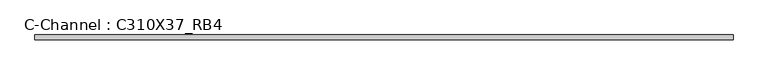
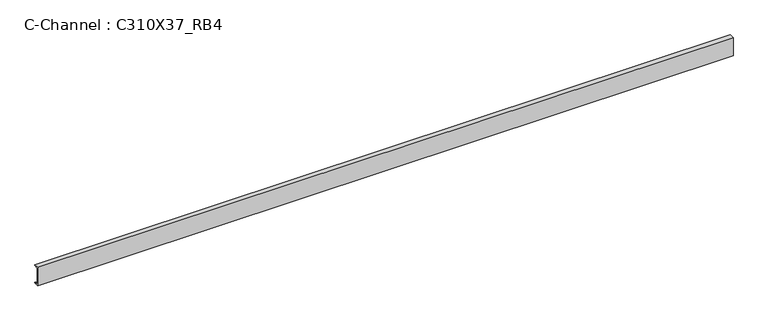
"""IFC4 building model written with IfcOpenShell, lengths in millimetres: beam geometry, C-Channel : C310X37_RB4."""

import ifcopenshell
import ifcopenshell.guid

model = None  # the IFC model being written
_history = None  # IfcOwnerHistory: only IFC2X3 demands one
_inside = {}  # id of a spatial element -> (the spatial element, [elements in it])
_under = {}  # id of a project, library or spatial element -> (it, [spatial elements below it])
_declared = {}  # id of a project -> (the project, [libraries it declares])
_typed = {}  # id of a type object -> (the type object, [elements of that type])
_made_of = {}  # id of a material, layer set ... -> (it, [elements and type objects made of it])


def new_model(schema):
    """Start an empty IFC model of exactly this schema.

    Asked for "IFC4X3", IfcOpenShell would pick the latest addendum, in which some entities
    have other attributes; the version numbers below select the first issue.
    IFC2X3 requires an IfcOwnerHistory on every rooted entity: one is made here for all.
    """
    global model, _history
    if schema == "IFC4X3":
        model = ifcopenshell.file(schema_version=(4, 3, 0, 0))
    else:
        model = ifcopenshell.file(schema=schema)
    _inside.clear()
    _under.clear()
    _declared.clear()
    _typed.clear()
    _made_of.clear()
    _history = None
    if model.schema == "IFC2X3":
        org = make("IfcOrganization", Name="unknown")
        user = make(
            "IfcPersonAndOrganization",
            ThePerson=make("IfcPerson", FamilyName="unknown"),
            TheOrganization=org,
        )
        app = make(
            "IfcApplication",
            ApplicationDeveloper=org,
            Version="unknown",
            ApplicationFullName="unknown",
            ApplicationIdentifier="unknown",
        )
        _history = make(
            "IfcOwnerHistory",
            OwningUser=user,
            OwningApplication=app,
            ChangeAction="ADDED",
            CreationDate=0,
        )
    return model


def make(cls, **values):
    """One entity of the class cls with the attributes given. An attribute that is None is left unset."""
    return model.create_entity(
        cls, **{name: value for name, value in values.items() if value is not None}
    )


def rooted(cls, **values):
    """An entity with a GlobalId (a new one), such as an element, a storey or a relation."""
    return make(cls, GlobalId=ifcopenshell.guid.new(), OwnerHistory=_history, **values)


def si_unit(unit_type, name, prefix=None):
    """IfcSIUnit, for example si_unit("LENGTHUNIT", "METRE", prefix="MILLI")."""
    return make("IfcSIUnit", UnitType=unit_type, Prefix=prefix, Name=name)


def assignment(units):
    """IfcUnitAssignment: the units of a project."""
    return None if units is None else make("IfcUnitAssignment", Units=units)


def point(xyz):
    """IfcCartesianPoint."""
    return None if xyz is None else make("IfcCartesianPoint", Coordinates=xyz)


def direction(xyz):
    """IfcDirection."""
    return None if xyz is None else make("IfcDirection", DirectionRatios=xyz)


def frame(location, z_axis=None, x_axis=None):
    """IfcAxis2Placement3D, a coordinate frame: its origin and axes. An axis left out is left unset."""
    return make(
        "IfcAxis2Placement3D",
        Location=point(location),
        Axis=direction(z_axis),
        RefDirection=direction(x_axis),
    )


def frame_2d(location, x_axis=None):
    """IfcAxis2Placement2D, a coordinate frame in the plane: its origin and x axis."""
    return make(
        "IfcAxis2Placement2D", Location=point(location), RefDirection=direction(x_axis)
    )


def origin():
    """The frame at (0, 0, 0) with its axes left unset."""
    return frame((0.0, 0.0, 0.0))


def place(relative_to, where):
    """IfcLocalPlacement: puts the frame where relative to a parent placement (None: the world)."""
    return make(
        "IfcLocalPlacement", PlacementRelTo=relative_to, RelativePlacement=where
    )


def context(
    kind, dimensions, precision=None, world=None, true_north=None, identifier=None
):
    """IfcGeometricRepresentationContext, for example the 3D "Model" context."""
    return make(
        "IfcGeometricRepresentationContext",
        ContextIdentifier=identifier,
        ContextType=kind,
        CoordinateSpaceDimension=dimensions,
        Precision=precision,
        WorldCoordinateSystem=world,
        TrueNorth=true_north,
    )


def project(units=None, contexts=None):
    """IfcProject with its units and contexts."""
    return rooted(
        "IfcProject",
        Name="project",
        RepresentationContexts=contexts,
        UnitsInContext=assignment(units),
    )


def spatial(cls, under=None, at=None, **own):
    """A site, building, storey or space (cls), placed at a placement, below another one or the project."""
    s = rooted(cls, ObjectPlacement=at, **own)
    if under is not None:
        _under.setdefault(under.id(), (under, []))[1].append(s)
    return s


def polyline(points):
    """IfcPolyline through the points."""
    return make("IfcPolyline", Points=[point(p) for p in points])


def circle_curve(where, radius):
    """IfcCircle in the frame where."""
    return make("IfcCircle", Position=where, Radius=radius)


def trimmed(basis, trim1, trim2, sense, master):
    """IfcTrimmedCurve: the piece of a basis curve between two trims."""
    return make(
        "IfcTrimmedCurve",
        BasisCurve=basis,
        Trim1=trim1,
        Trim2=trim2,
        SenseAgreement=sense,
        MasterRepresentation=master,
    )


def segment(curve, same_sense, transition):
    """IfcCompositeCurveSegment."""
    return make(
        "IfcCompositeCurveSegment",
        Transition=transition,
        SameSense=same_sense,
        ParentCurve=curve,
    )


def composite_curve(segments, self_intersect=None):
    """IfcCompositeCurve: segments joined end to end."""
    return make("IfcCompositeCurve", Segments=segments, SelfIntersect=self_intersect)


def outline(outer, holes=None, kind="AREA"):
    """IfcArbitraryClosedProfileDef: a profile drawn as a closed curve; with holes, ...WithVoids."""
    if holes is None:
        return make("IfcArbitraryClosedProfileDef", ProfileType=kind, OuterCurve=outer)
    return make(
        "IfcArbitraryProfileDefWithVoids",
        ProfileType=kind,
        OuterCurve=outer,
        InnerCurves=holes,
    )


def extrude(swept, where, along, depth):
    """IfcExtrudedAreaSolid: the profile swept, set in the frame where, extruded along a direction by depth."""
    return make(
        "IfcExtrudedAreaSolid",
        SweptArea=swept,
        Position=where,
        ExtrudedDirection=direction(along),
        Depth=depth,
    )


def shape(context_of_items, identifier, shape_type, items):
    """IfcShapeRepresentation: the items that make up one representation, for example the "Body"."""
    return make(
        "IfcShapeRepresentation",
        ContextOfItems=context_of_items,
        RepresentationIdentifier=identifier,
        RepresentationType=shape_type,
        Items=items,
    )


def source(mapping_origin, context_of_items, identifier, shape_type, items):
    """IfcRepresentationMap: a shape defined once, which mapped items show again and again."""
    return make(
        "IfcRepresentationMap",
        MappingOrigin=mapping_origin,
        MappedRepresentation=shape(context_of_items, identifier, shape_type, items),
    )


def transform(
    local_origin,
    x_axis=None,
    y_axis=None,
    z_axis=None,
    scale=None,
    scale2=None,
    scale3=None,
    uniform=True,
):
    """IfcCartesianTransformationOperator3D, or its non-uniform kind. x_axis, y_axis, z_axis: its Axis1, 2, 3."""
    if uniform:
        return make(
            "IfcCartesianTransformationOperator3D",
            Axis1=direction(x_axis),
            Axis2=direction(y_axis),
            LocalOrigin=point(local_origin),
            Scale=scale,
            Axis3=direction(z_axis),
        )
    return make(
        "IfcCartesianTransformationOperator3DnonUniform",
        Axis1=direction(x_axis),
        Axis2=direction(y_axis),
        LocalOrigin=point(local_origin),
        Scale=scale,
        Axis3=direction(z_axis),
        Scale2=scale2,
        Scale3=scale3,
    )


def mapped(mapping_source, mapping_target):
    """IfcMappedItem: shows the shape of a source again, moved by a transform."""
    return make(
        "IfcMappedItem", MappingSource=mapping_source, MappingTarget=mapping_target
    )


def made_of(thing, what):
    """Note that an element or type object is made of a material, layer set ...; save() writes the relation."""
    if what is not None:
        _made_of.setdefault(what.id(), (what, []))[1].append(thing)
    return thing


def element(
    cls,
    number,
    at=None,
    inside=None,
    cuts=None,
    type_object=None,
    material=None,
    context=None,
    identifier="Body",
    shape_type=None,
    held_by="IfcProductDefinitionShape",
    body=None,
    shapes=None,
    **own,
):
    """One element of the class cls, such as IfcWall. Its Tag is "e" and its number.

    at: its placement. inside: the storey or other place that contains it. cuts: it is an
    opening in that element (IfcRelVoidsElement). A single representation is given by context,
    identifier, shape_type and body (its items); several are given by shapes. held_by: the class
    of the entity that holds the representations. save() writes the other relations.
    """
    e = rooted(cls, Tag="e%d" % number, ObjectPlacement=at, **own)
    if body is not None:
        shapes = [shape(context, identifier, shape_type, body)]
    if shapes is not None:
        e.Representation = make(held_by, Representations=shapes)
    if inside is not None:
        _inside.setdefault(inside.id(), (inside, []))[1].append(e)
    if cuts is not None:
        rooted(
            "IfcRelVoidsElement", RelatingBuildingElement=cuts, RelatedOpeningElement=e
        )
    if type_object is not None:
        _typed.setdefault(type_object.id(), (type_object, []))[1].append(e)
    return made_of(e, material)


def aggregate(whole, parts):
    """IfcRelAggregates: a whole, such as a stair, and the parts it consists of."""
    return rooted("IfcRelAggregates", RelatingObject=whole, RelatedObjects=parts)


def save(model, path):
    """Write the relations noted so far, then the file.

    IfcRelAggregates (storeys below a building ...), IfcRelContainedInSpatialStructure (elements
    in a storey), IfcRelDefinesByType, IfcRelAssociatesMaterial and IfcRelDeclares: one each for
    every whole, place, type object, material and project.
    """
    for whole, parts in _under.values():
        aggregate(whole, parts)
    for where, things in _inside.values():
        rooted(
            "IfcRelContainedInSpatialStructure",
            RelatedElements=things,
            RelatingStructure=where,
        )
    for kind, things in _typed.values():
        rooted("IfcRelDefinesByType", RelatedObjects=things, RelatingType=kind)
    for what, things in _made_of.values():
        rooted("IfcRelAssociatesMaterial", RelatedObjects=things, RelatingMaterial=what)
    for by, libraries in _declared.values():
        rooted("IfcRelDeclares", RelatingContext=by, RelatedDefinitions=libraries)
    model.write(path)


def c_channel_c310x37_rb4_3b9980a8(model_context):
    return source(origin(), model_context, "Body", "SweptSolid", [
        extrude(outline(composite_curve([segment(polyline([(-17.1196, 152.4), (60.3504, 152.4)]), True, "CONTINUOUS"), segment(trimmed(circle_curve(frame_2d((47.625, 152.4)), 12.7254), [point((60.3504, 152.4))], [point((47.625, 139.6746))], False, "CARTESIAN"), True, "CONTINUOUS"), segment(polyline([(47.625, 139.6746), (-7.2898, 130.9769501), (-7.2898, -130.9769501), (47.625, -139.6746)]), True, "CONTINUOUS"), segment(trimmed(circle_curve(frame_2d((47.625, -152.4)), 12.7254), [point((47.625, -139.6746))], [point((60.3504, -152.4))], False, "CARTESIAN"), True, "CONTINUOUS"), segment(polyline([(60.3504, -152.4), (-17.1196, -152.4), (-17.1196, 152.4)]), True, "CONTINUOUS")], self_intersect=False)), frame((-5538.3209452, 0.0, 0.0), z_axis=(1.0, 0.0, 0.0), x_axis=(0.0, 1.0, 0.0)), (0.0, 0.0, 1.0), 11055.4234616),
    ])


if __name__ == "__main__":
    model = new_model("IFC4")
    model_context = context("Model", 3, world=origin())
    ifc_project = project(units=[si_unit("LENGTHUNIT", "METRE", prefix="MILLI")], contexts=[model_context])
    site = spatial("IfcSite", under=ifc_project)
    building = spatial("IfcBuilding", under=site)
    placement = place(None, origin())
    c_channel_c310x37_rb4_shape = c_channel_c310x37_rb4_3b9980a8(model_context)
    element("IfcBeam", 1, ObjectType="C-Channel : C310X37_RB4", at=placement, inside=building, context=model_context, shape_type="MappedRepresentation", body=[
        mapped(c_channel_c310x37_rb4_shape, transform((0.0, 0.0, 0.0), x_axis=(1.0, 0.0, 0.0), y_axis=(0.0, 1.0, 0.0), z_axis=(0.0, 0.0, 1.0))),
    ])
    save(model, "model.ifc")

# Revit data of these elements
# Type "C-Channel : C310X37_RB4"
#   Assembly Code = "B10"
#   W = 25
#   Length [instance default] = 1524 mm
#   bf = 77.47 mm
#   d = 304.8 mm
#   tf = 12.725 mm
#   tw = 9.83 mm
#   x = 17.12 mm
#   A = 0.00473547 m²
#   Structural Material [instance default] = Steel ASTM A36
# Element 1 (IfcBeam, "C-Channel : C310X37_RB4")
#   Structural Material = Steel ASTM A992
#   Materials on its faces: "Steel ASTM A992"
# Materials
#   "Steel ASTM A36": class "Metal", colour RGB 199 199 199, transparency 0, Description = "Structural steel, ASTM A36 Grade B, mill finish", Cost = 0
#   "Steel ASTM A992": class "Metal", colour RGB 199 199 199, transparency 0, Description = "Structural steel 50ksi", Cost = 0
